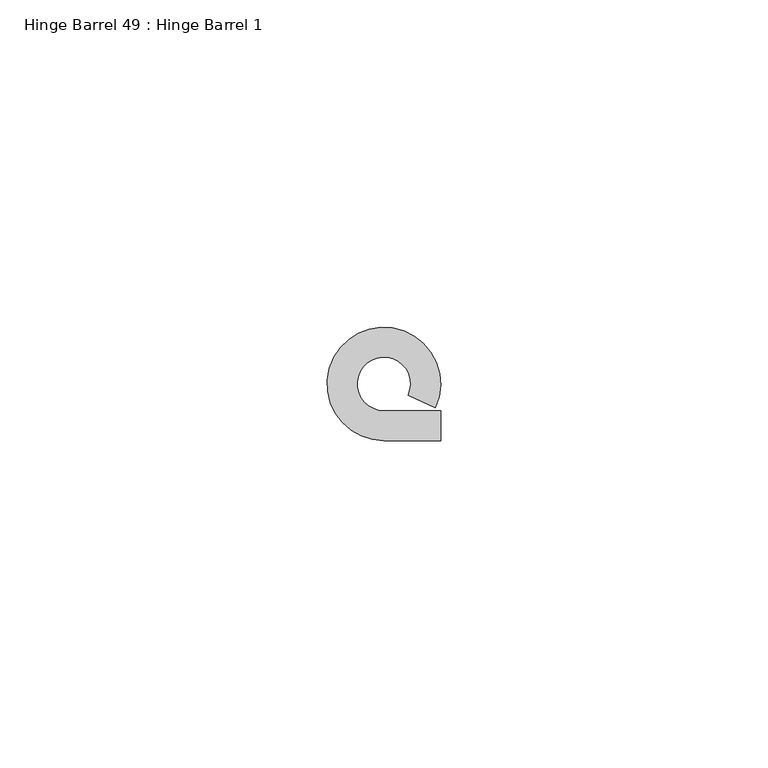
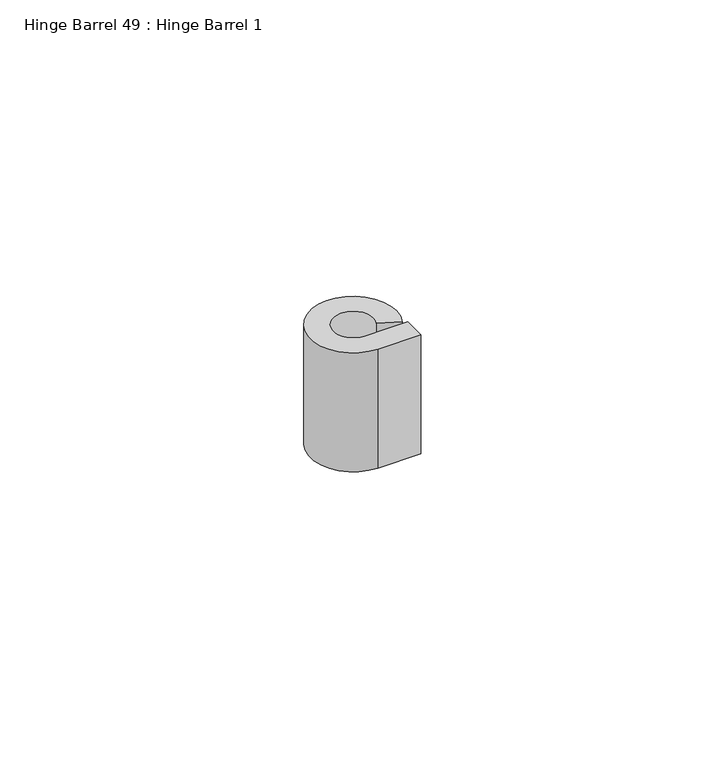
"""IFC4 building model written with IfcOpenShell, lengths in millimetres: proxy geometry, Hinge Barrel 49 : Hinge Barrel 1."""

from ifc_helpers import new_model, si_unit, point, frame, frame_2d, origin, place, context, project, spatial, polyline, circle_curve, trimmed, segment, composite_curve, outline, extrude, source, transform, mapped, element, save


def hinge_barrel_49_hinge_barrel_1_b6c159eb(model_context):
    return source(origin(), model_context, "Body", "SweptSolid", [
        extrude(outline(composite_curve([segment(polyline([(587323.2214739, -534104.7943841), (587327.7934739, -534104.7943841), (587327.7934739, -534109.3584466), (587319.1320739, -534109.3584466)]), True, "CONTINUOUS"), segment(trimmed(circle_curve(frame_2d((587319.1320739, -534100.7049841)), 8.6534625), [point((587319.1320739, -534109.3584466))], [point((587326.986084, -534104.3377433))], False, "CARTESIAN"), True, "CONTINUOUS"), segment(polyline([(587326.986084, -534104.3377433), (587322.8436736, -534102.421731)]), True, "CONTINUOUS"), segment(trimmed(circle_curve(frame_2d((587319.1320739, -534100.7049841)), 4.0894), [point((587322.8436736, -534102.421731))], [point((587319.1320739, -534104.7943841))], True, "CARTESIAN"), True, "CONTINUOUS"), segment(polyline([(587319.1320739, -534104.7943841), (587323.2214739, -534104.7943841)]), True, "CONTINUOUS")], self_intersect=False)), frame((0.0, 0.0, 1123.95), z_axis=(0.0, 0.0, 1.0), x_axis=(1.0, 0.0, 0.0)), (0.0, 0.0, 1.0), 25.4),
    ])


if __name__ == "__main__":
    model = new_model("IFC4")
    model_context = context("Model", 3, world=origin())
    ifc_project = project(units=[si_unit("LENGTHUNIT", "METRE", prefix="MILLI")], contexts=[model_context])
    site = spatial("IfcSite", under=ifc_project)
    building = spatial("IfcBuilding", under=site)
    placement = place(None, origin())
    hinge_barrel_49_hinge_barrel_1_shape = hinge_barrel_49_hinge_barrel_1_b6c159eb(model_context)
    element("IfcBuildingElementProxy", 1, Name="Hinge Barrel 49 : Hinge Barrel 1", ObjectType="Hinge Barrel 49 : Hinge Barrel 1", at=placement, inside=building, context=model_context, shape_type="MappedRepresentation", body=[
        mapped(hinge_barrel_49_hinge_barrel_1_shape, transform((0.0, 0.0, 0.0), x_axis=(1.0, 0.0, 0.0), y_axis=(0.0, 1.0, 0.0), z_axis=(0.0, 0.0, 1.0))),
    ])
    save(model, "model.ifc")

# Revit data of these elements
# Element 1 (IfcBuildingElementProxy, "Hinge Barrel 49 : Hinge Barrel 1")
#   Materials on its faces: "6\"X6\" WELD-ON STL BUTT HINGE"
# Materials
#   "6\"X6\" WELD-ON STL BUTT HINGE": class "Metal", colour RGB 189 187 185, transparency 0, Description = "Carbon steel", Cost = 0
